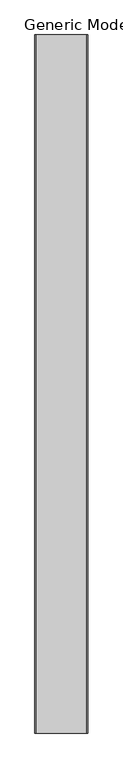
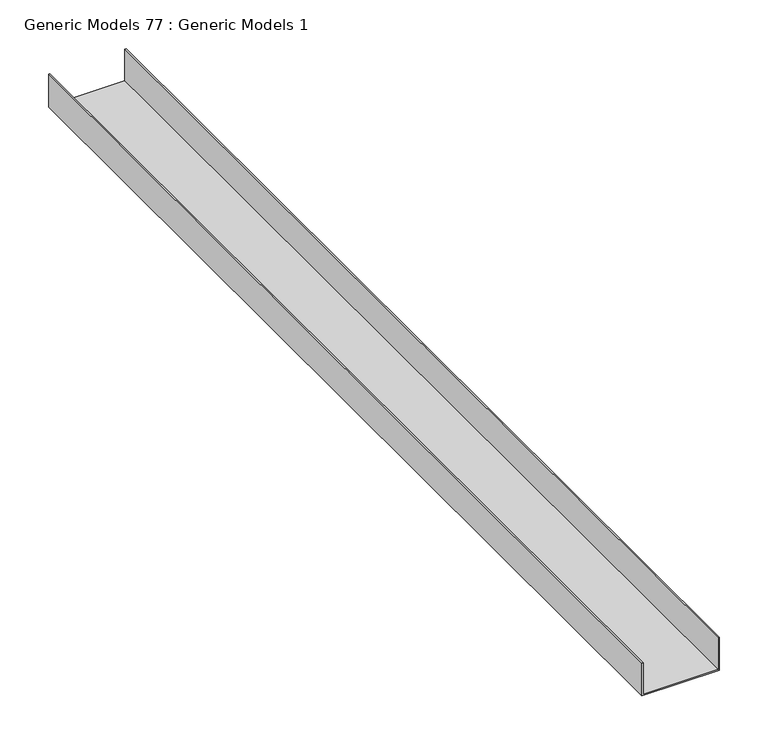
"""IFC4 building model written with IfcOpenShell, lengths in millimetres: proxy geometry, Generic Models 77 : Generic Models 1."""

from ifc_helpers import new_model, si_unit, frame, origin, place, context, project, spatial, polyline, outline, extrude, source, transform, mapped, element, save


def generic_models_77_generic_models_1_bf0b6e5f(model_context):
    return source(origin(), model_context, "Body", "SweptSolid", [
        extrude(outline(polyline([(-2150.4233876, 49802.3181639), (-2109.1483876, 49802.3181639), (-2109.1483876, 49800.7306639), (-2148.8358876, 49800.7306639), (-2148.8358876, 49711.8306639), (-2109.1483876, 49711.8306639), (-2109.1483876, 49710.2431639), (-2150.4233876, 49710.2431639), (-2150.4233876, 49802.3181639)])), frame((0.0, 0.0, 0.0), z_axis=(0.0, 1.0, 0.0), x_axis=(0.0, 0.0, 1.0)), (0.0, 0.0, 1.0), 1219.2),
    ])


if __name__ == "__main__":
    model = new_model("IFC4")
    model_context = context("Model", 3, world=origin())
    ifc_project = project(units=[si_unit("LENGTHUNIT", "METRE", prefix="MILLI")], contexts=[model_context])
    site = spatial("IfcSite", under=ifc_project)
    building = spatial("IfcBuilding", under=site)
    placement = place(None, origin())
    generic_models_77_generic_models_1_shape = generic_models_77_generic_models_1_bf0b6e5f(model_context)
    element("IfcBuildingElementProxy", 1, Name="Generic Models 77 : Generic Models 1", ObjectType="Generic Models 77 : Generic Models 1", at=placement, inside=building, context=model_context, shape_type="MappedRepresentation", body=[
        mapped(generic_models_77_generic_models_1_shape, transform((0.0, 0.0, 0.0), x_axis=(1.0, 0.0, 0.0), y_axis=(0.0, 1.0, 0.0), z_axis=(0.0, 0.0, 1.0))),
    ])
    save(model, "model.ifc")

# Revit data of these elements
# Element 1 (IfcBuildingElementProxy, "Generic Models 77 : Generic Models 1")
#   Materials on its faces: "METAL RUNNER CHANNEL; FASTEN @ 24\" O.C."
# Materials
#   "METAL RUNNER CHANNEL; FASTEN @ 24\" O.C.": class "Unassigned", colour RGB 210 209 208, transparency 0, Keynote = "M05121300.02", Cost = 0
